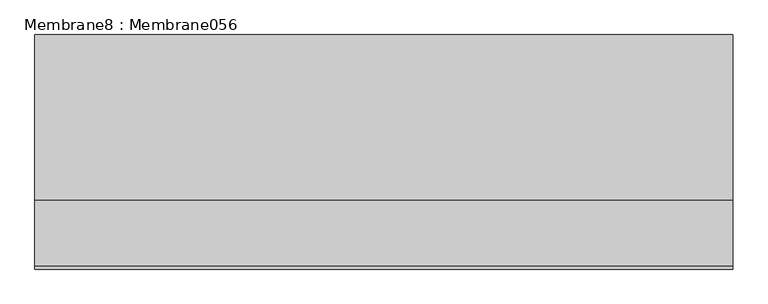
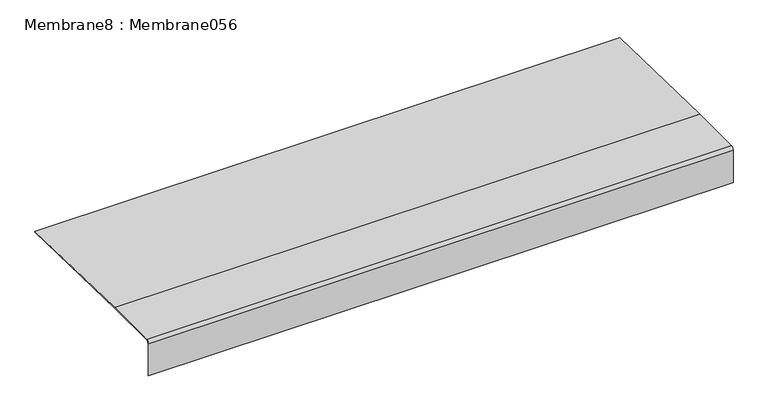
"""IFC4 building model written with IfcOpenShell, lengths in millimetres: proxy geometry, Membrane8 : Membrane056."""

import ifcopenshell
import ifcopenshell.guid

model = None  # the IFC model being written
_history = None  # IfcOwnerHistory: only IFC2X3 demands one
_inside = {}  # id of a spatial element -> (the spatial element, [elements in it])
_under = {}  # id of a project, library or spatial element -> (it, [spatial elements below it])
_declared = {}  # id of a project -> (the project, [libraries it declares])
_typed = {}  # id of a type object -> (the type object, [elements of that type])
_made_of = {}  # id of a material, layer set ... -> (it, [elements and type objects made of it])


def new_model(schema):
    """Start an empty IFC model of exactly this schema.

    Asked for "IFC4X3", IfcOpenShell would pick the latest addendum, in which some entities
    have other attributes; the version numbers below select the first issue.
    IFC2X3 requires an IfcOwnerHistory on every rooted entity: one is made here for all.
    """
    global model, _history
    if schema == "IFC4X3":
        model = ifcopenshell.file(schema_version=(4, 3, 0, 0))
    else:
        model = ifcopenshell.file(schema=schema)
    _inside.clear()
    _under.clear()
    _declared.clear()
    _typed.clear()
    _made_of.clear()
    _history = None
    if model.schema == "IFC2X3":
        org = make("IfcOrganization", Name="unknown")
        user = make(
            "IfcPersonAndOrganization",
            ThePerson=make("IfcPerson", FamilyName="unknown"),
            TheOrganization=org,
        )
        app = make(
            "IfcApplication",
            ApplicationDeveloper=org,
            Version="unknown",
            ApplicationFullName="unknown",
            ApplicationIdentifier="unknown",
        )
        _history = make(
            "IfcOwnerHistory",
            OwningUser=user,
            OwningApplication=app,
            ChangeAction="ADDED",
            CreationDate=0,
        )
    return model


def make(cls, **values):
    """One entity of the class cls with the attributes given. An attribute that is None is left unset."""
    return model.create_entity(
        cls, **{name: value for name, value in values.items() if value is not None}
    )


def rooted(cls, **values):
    """An entity with a GlobalId (a new one), such as an element, a storey or a relation."""
    return make(cls, GlobalId=ifcopenshell.guid.new(), OwnerHistory=_history, **values)


def si_unit(unit_type, name, prefix=None):
    """IfcSIUnit, for example si_unit("LENGTHUNIT", "METRE", prefix="MILLI")."""
    return make("IfcSIUnit", UnitType=unit_type, Prefix=prefix, Name=name)


def assignment(units):
    """IfcUnitAssignment: the units of a project."""
    return None if units is None else make("IfcUnitAssignment", Units=units)


def point(xyz):
    """IfcCartesianPoint."""
    return None if xyz is None else make("IfcCartesianPoint", Coordinates=xyz)


def direction(xyz):
    """IfcDirection."""
    return None if xyz is None else make("IfcDirection", DirectionRatios=xyz)


def frame(location, z_axis=None, x_axis=None):
    """IfcAxis2Placement3D, a coordinate frame: its origin and axes. An axis left out is left unset."""
    return make(
        "IfcAxis2Placement3D",
        Location=point(location),
        Axis=direction(z_axis),
        RefDirection=direction(x_axis),
    )


def frame_2d(location, x_axis=None):
    """IfcAxis2Placement2D, a coordinate frame in the plane: its origin and x axis."""
    return make(
        "IfcAxis2Placement2D", Location=point(location), RefDirection=direction(x_axis)
    )


def origin():
    """The frame at (0, 0, 0) with its axes left unset."""
    return frame((0.0, 0.0, 0.0))


def place(relative_to, where):
    """IfcLocalPlacement: puts the frame where relative to a parent placement (None: the world)."""
    return make(
        "IfcLocalPlacement", PlacementRelTo=relative_to, RelativePlacement=where
    )


def context(
    kind, dimensions, precision=None, world=None, true_north=None, identifier=None
):
    """IfcGeometricRepresentationContext, for example the 3D "Model" context."""
    return make(
        "IfcGeometricRepresentationContext",
        ContextIdentifier=identifier,
        ContextType=kind,
        CoordinateSpaceDimension=dimensions,
        Precision=precision,
        WorldCoordinateSystem=world,
        TrueNorth=true_north,
    )


def project(units=None, contexts=None):
    """IfcProject with its units and contexts."""
    return rooted(
        "IfcProject",
        Name="project",
        RepresentationContexts=contexts,
        UnitsInContext=assignment(units),
    )


def spatial(cls, under=None, at=None, **own):
    """A site, building, storey or space (cls), placed at a placement, below another one or the project."""
    s = rooted(cls, ObjectPlacement=at, **own)
    if under is not None:
        _under.setdefault(under.id(), (under, []))[1].append(s)
    return s


def polyline(points):
    """IfcPolyline through the points."""
    return make("IfcPolyline", Points=[point(p) for p in points])


def circle_curve(where, radius):
    """IfcCircle in the frame where."""
    return make("IfcCircle", Position=where, Radius=radius)


def trimmed(basis, trim1, trim2, sense, master):
    """IfcTrimmedCurve: the piece of a basis curve between two trims."""
    return make(
        "IfcTrimmedCurve",
        BasisCurve=basis,
        Trim1=trim1,
        Trim2=trim2,
        SenseAgreement=sense,
        MasterRepresentation=master,
    )


def segment(curve, same_sense, transition):
    """IfcCompositeCurveSegment."""
    return make(
        "IfcCompositeCurveSegment",
        Transition=transition,
        SameSense=same_sense,
        ParentCurve=curve,
    )


def composite_curve(segments, self_intersect=None):
    """IfcCompositeCurve: segments joined end to end."""
    return make("IfcCompositeCurve", Segments=segments, SelfIntersect=self_intersect)


def outline(outer, holes=None, kind="AREA"):
    """IfcArbitraryClosedProfileDef: a profile drawn as a closed curve; with holes, ...WithVoids."""
    if holes is None:
        return make("IfcArbitraryClosedProfileDef", ProfileType=kind, OuterCurve=outer)
    return make(
        "IfcArbitraryProfileDefWithVoids",
        ProfileType=kind,
        OuterCurve=outer,
        InnerCurves=holes,
    )


def extrude(swept, where, along, depth):
    """IfcExtrudedAreaSolid: the profile swept, set in the frame where, extruded along a direction by depth."""
    return make(
        "IfcExtrudedAreaSolid",
        SweptArea=swept,
        Position=where,
        ExtrudedDirection=direction(along),
        Depth=depth,
    )


def shape(context_of_items, identifier, shape_type, items):
    """IfcShapeRepresentation: the items that make up one representation, for example the "Body"."""
    return make(
        "IfcShapeRepresentation",
        ContextOfItems=context_of_items,
        RepresentationIdentifier=identifier,
        RepresentationType=shape_type,
        Items=items,
    )


def source(mapping_origin, context_of_items, identifier, shape_type, items):
    """IfcRepresentationMap: a shape defined once, which mapped items show again and again."""
    return make(
        "IfcRepresentationMap",
        MappingOrigin=mapping_origin,
        MappedRepresentation=shape(context_of_items, identifier, shape_type, items),
    )


def transform(
    local_origin,
    x_axis=None,
    y_axis=None,
    z_axis=None,
    scale=None,
    scale2=None,
    scale3=None,
    uniform=True,
):
    """IfcCartesianTransformationOperator3D, or its non-uniform kind. x_axis, y_axis, z_axis: its Axis1, 2, 3."""
    if uniform:
        return make(
            "IfcCartesianTransformationOperator3D",
            Axis1=direction(x_axis),
            Axis2=direction(y_axis),
            LocalOrigin=point(local_origin),
            Scale=scale,
            Axis3=direction(z_axis),
        )
    return make(
        "IfcCartesianTransformationOperator3DnonUniform",
        Axis1=direction(x_axis),
        Axis2=direction(y_axis),
        LocalOrigin=point(local_origin),
        Scale=scale,
        Axis3=direction(z_axis),
        Scale2=scale2,
        Scale3=scale3,
    )


def mapped(mapping_source, mapping_target):
    """IfcMappedItem: shows the shape of a source again, moved by a transform."""
    return make(
        "IfcMappedItem", MappingSource=mapping_source, MappingTarget=mapping_target
    )


def made_of(thing, what):
    """Note that an element or type object is made of a material, layer set ...; save() writes the relation."""
    if what is not None:
        _made_of.setdefault(what.id(), (what, []))[1].append(thing)
    return thing


def element(
    cls,
    number,
    at=None,
    inside=None,
    cuts=None,
    type_object=None,
    material=None,
    context=None,
    identifier="Body",
    shape_type=None,
    held_by="IfcProductDefinitionShape",
    body=None,
    shapes=None,
    **own,
):
    """One element of the class cls, such as IfcWall. Its Tag is "e" and its number.

    at: its placement. inside: the storey or other place that contains it. cuts: it is an
    opening in that element (IfcRelVoidsElement). A single representation is given by context,
    identifier, shape_type and body (its items); several are given by shapes. held_by: the class
    of the entity that holds the representations. save() writes the other relations.
    """
    e = rooted(cls, Tag="e%d" % number, ObjectPlacement=at, **own)
    if body is not None:
        shapes = [shape(context, identifier, shape_type, body)]
    if shapes is not None:
        e.Representation = make(held_by, Representations=shapes)
    if inside is not None:
        _inside.setdefault(inside.id(), (inside, []))[1].append(e)
    if cuts is not None:
        rooted(
            "IfcRelVoidsElement", RelatingBuildingElement=cuts, RelatedOpeningElement=e
        )
    if type_object is not None:
        _typed.setdefault(type_object.id(), (type_object, []))[1].append(e)
    return made_of(e, material)


def aggregate(whole, parts):
    """IfcRelAggregates: a whole, such as a stair, and the parts it consists of."""
    return rooted("IfcRelAggregates", RelatingObject=whole, RelatedObjects=parts)


def save(model, path):
    """Write the relations noted so far, then the file.

    IfcRelAggregates (storeys below a building ...), IfcRelContainedInSpatialStructure (elements
    in a storey), IfcRelDefinesByType, IfcRelAssociatesMaterial and IfcRelDeclares: one each for
    every whole, place, type object, material and project.
    """
    for whole, parts in _under.values():
        aggregate(whole, parts)
    for where, things in _inside.values():
        rooted(
            "IfcRelContainedInSpatialStructure",
            RelatedElements=things,
            RelatingStructure=where,
        )
    for kind, things in _typed.values():
        rooted("IfcRelDefinesByType", RelatedObjects=things, RelatingType=kind)
    for what, things in _made_of.values():
        rooted("IfcRelAssociatesMaterial", RelatedObjects=things, RelatingMaterial=what)
    for by, libraries in _declared.values():
        rooted("IfcRelDeclares", RelatingContext=by, RelatedDefinitions=libraries)
    model.write(path)


def membrane8_membrane056_cd553bbe(model_context):
    return source(origin(), model_context, "Body", "SweptSolid", [
        extrude(outline(composite_curve([segment(polyline([(-5544.5374023, 40101.8965244), (-5546.5374023, 40101.8965244), (-5546.5374023, 40218.6165225)]), True, "CONTINUOUS"), segment(trimmed(circle_curve(frame_2d((-5536.5374023, 40218.6165225)), 10.0), [point((-5546.5374023, 40218.6165225))], [point((-5536.5374023, 40228.6165225))], False, "CARTESIAN"), True, "CONTINUOUS"), segment(polyline([(-5536.5374023, 40228.6165225), (-5348.0337978, 40228.6165225), (-4874.4404297, 40217.78125), (-4874.4861754, 40215.7817732), (-5348.0566737, 40226.6165225), (-5536.5374023, 40226.6165225)]), True, "CONTINUOUS"), segment(trimmed(circle_curve(frame_2d((-5536.5374023, 40218.6165225)), 8.0), [point((-5536.5374023, 40226.6165225))], [point((-5544.5374023, 40218.6165225))], True, "CARTESIAN"), True, "CONTINUOUS"), segment(polyline([(-5544.5374023, 40218.6165225), (-5544.5374023, 40101.8965244)]), True, "CONTINUOUS")], self_intersect=False)), frame((12383.0178845, 0.0, 0.0), z_axis=(1.0, 0.0, 0.0), x_axis=(0.0, 1.0, 0.0)), (0.0, 0.0, 1.0), 2000.0),
    ])


if __name__ == "__main__":
    model = new_model("IFC4")
    model_context = context("Model", 3, world=origin())
    ifc_project = project(units=[si_unit("LENGTHUNIT", "METRE", prefix="MILLI")], contexts=[model_context])
    site = spatial("IfcSite", under=ifc_project)
    building = spatial("IfcBuilding", under=site)
    placement = place(None, origin())
    membrane8_membrane056_shape = membrane8_membrane056_cd553bbe(model_context)
    element("IfcBuildingElementProxy", 1, Name="Membrane8 : Membrane056", ObjectType="Membrane8 : Membrane056", at=placement, inside=building, context=model_context, shape_type="MappedRepresentation", body=[
        mapped(membrane8_membrane056_shape, transform((0.0, 0.0, 0.0), x_axis=(1.0, 0.0, 0.0), y_axis=(0.0, 1.0, 0.0), z_axis=(0.0, 0.0, 1.0))),
    ])
    save(model, "model.ifc")

# Revit data of these elements
# Type "Membrane8 : Membrane056"
#   NameOverride = "Membrane056"
# Element 1 (IfcBuildingElementProxy, "Membrane8 : Membrane056")
#   Materials on its faces: "THREE PLY BUILT UP ROOF MEMBRANE"
# Materials
#   "THREE PLY BUILT UP ROOF MEMBRANE": class "Unassigned", colour RGB 63 63 63, transparency 0
